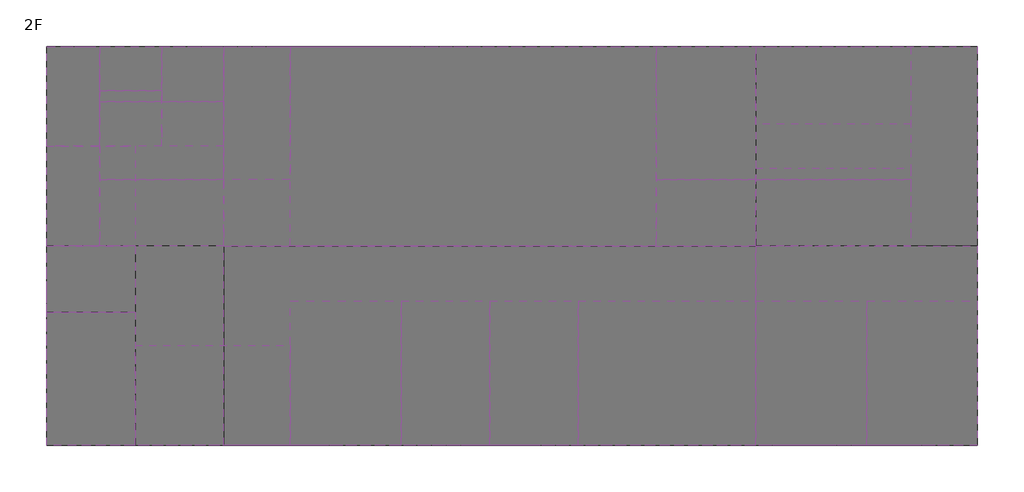
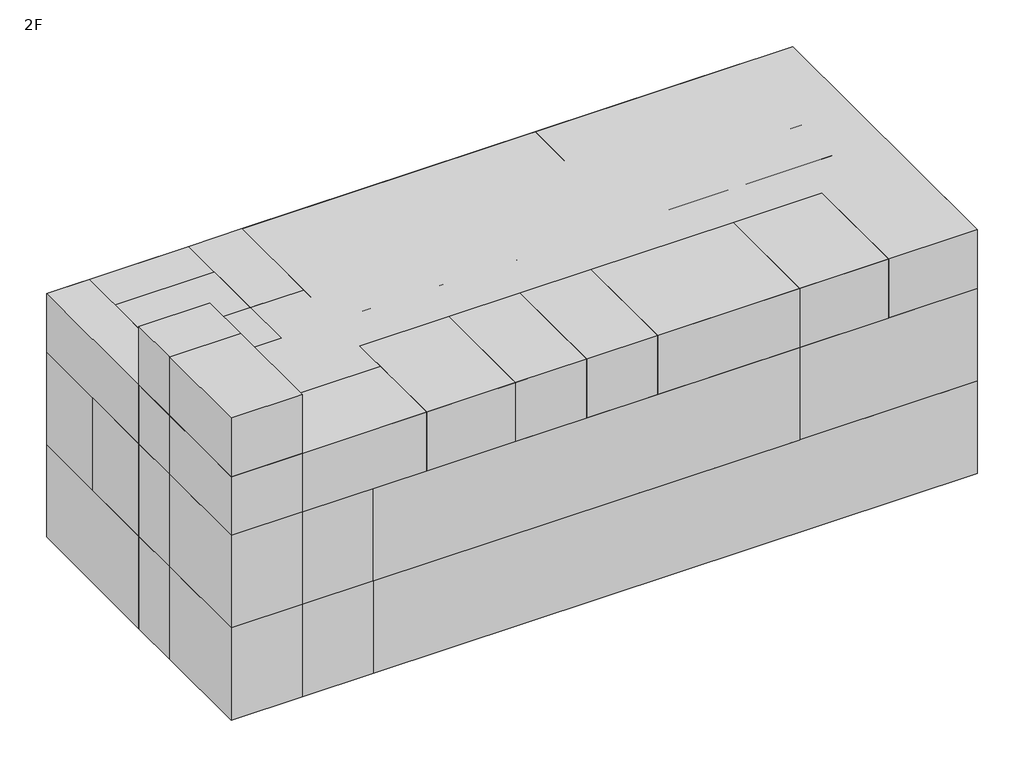
# One storey: 39 proxies.
"""IFC4 building model written with IfcOpenShell, lengths in millimetres."""

import ifcopenshell
import ifcopenshell.guid

model = None  # the IFC model being written
_history = None  # IfcOwnerHistory: only IFC2X3 demands one
_inside = {}  # id of a spatial element -> (the spatial element, [elements in it])
_under = {}  # id of a project, library or spatial element -> (it, [spatial elements below it])
_declared = {}  # id of a project -> (the project, [libraries it declares])
_typed = {}  # id of a type object -> (the type object, [elements of that type])
_made_of = {}  # id of a material, layer set ... -> (it, [elements and type objects made of it])


def new_model(schema):
    """Start an empty IFC model of exactly this schema.

    Asked for "IFC4X3", IfcOpenShell would pick the latest addendum, in which some entities
    have other attributes; the version numbers below select the first issue.
    IFC2X3 requires an IfcOwnerHistory on every rooted entity: one is made here for all.
    """
    global model, _history
    if schema == "IFC4X3":
        model = ifcopenshell.file(schema_version=(4, 3, 0, 0))
    else:
        model = ifcopenshell.file(schema=schema)
    _inside.clear()
    _under.clear()
    _declared.clear()
    _typed.clear()
    _made_of.clear()
    _history = None
    if model.schema == "IFC2X3":
        org = make("IfcOrganization", Name="unknown")
        user = make(
            "IfcPersonAndOrganization",
            ThePerson=make("IfcPerson", FamilyName="unknown"),
            TheOrganization=org,
        )
        app = make(
            "IfcApplication",
            ApplicationDeveloper=org,
            Version="unknown",
            ApplicationFullName="unknown",
            ApplicationIdentifier="unknown",
        )
        _history = make(
            "IfcOwnerHistory",
            OwningUser=user,
            OwningApplication=app,
            ChangeAction="ADDED",
            CreationDate=0,
        )
    return model


def make(cls, **values):
    """One entity of the class cls with the attributes given. An attribute that is None is left unset."""
    return model.create_entity(
        cls, **{name: value for name, value in values.items() if value is not None}
    )


def rooted(cls, **values):
    """An entity with a GlobalId (a new one), such as an element, a storey or a relation."""
    return make(cls, GlobalId=ifcopenshell.guid.new(), OwnerHistory=_history, **values)


def si_unit(unit_type, name, prefix=None):
    """IfcSIUnit, for example si_unit("LENGTHUNIT", "METRE", prefix="MILLI")."""
    return make("IfcSIUnit", UnitType=unit_type, Prefix=prefix, Name=name)


def assignment(units):
    """IfcUnitAssignment: the units of a project."""
    return None if units is None else make("IfcUnitAssignment", Units=units)


def point(xyz):
    """IfcCartesianPoint."""
    return None if xyz is None else make("IfcCartesianPoint", Coordinates=xyz)


def direction(xyz):
    """IfcDirection."""
    return None if xyz is None else make("IfcDirection", DirectionRatios=xyz)


def frame(location, z_axis=None, x_axis=None):
    """IfcAxis2Placement3D, a coordinate frame: its origin and axes. An axis left out is left unset."""
    return make(
        "IfcAxis2Placement3D",
        Location=point(location),
        Axis=direction(z_axis),
        RefDirection=direction(x_axis),
    )


def origin():
    """The frame at (0, 0, 0) with its axes left unset."""
    return frame((0.0, 0.0, 0.0))


def origin_with_axes():
    """The frame at (0, 0, 0) with the z axis (0, 0, 1) and the x axis (1, 0, 0) written out."""
    return frame((0.0, 0.0, 0.0), z_axis=(0.0, 0.0, 1.0), x_axis=(1.0, 0.0, 0.0))


def place(relative_to, where):
    """IfcLocalPlacement: puts the frame where relative to a parent placement (None: the world)."""
    return make(
        "IfcLocalPlacement", PlacementRelTo=relative_to, RelativePlacement=where
    )


def context(
    kind, dimensions, precision=None, world=None, true_north=None, identifier=None
):
    """IfcGeometricRepresentationContext, for example the 3D "Model" context."""
    return make(
        "IfcGeometricRepresentationContext",
        ContextIdentifier=identifier,
        ContextType=kind,
        CoordinateSpaceDimension=dimensions,
        Precision=precision,
        WorldCoordinateSystem=world,
        TrueNorth=true_north,
    )


def project(units=None, contexts=None):
    """IfcProject with its units and contexts."""
    return rooted(
        "IfcProject",
        Name="project",
        RepresentationContexts=contexts,
        UnitsInContext=assignment(units),
    )


def spatial(cls, under=None, at=None, **own):
    """A site, building, storey or space (cls), placed at a placement, below another one or the project."""
    s = rooted(cls, ObjectPlacement=at, **own)
    if under is not None:
        _under.setdefault(under.id(), (under, []))[1].append(s)
    return s


def polyline(points):
    """IfcPolyline through the points."""
    return make("IfcPolyline", Points=[point(p) for p in points])


def outline(outer, holes=None, kind="AREA"):
    """IfcArbitraryClosedProfileDef: a profile drawn as a closed curve; with holes, ...WithVoids."""
    if holes is None:
        return make("IfcArbitraryClosedProfileDef", ProfileType=kind, OuterCurve=outer)
    return make(
        "IfcArbitraryProfileDefWithVoids",
        ProfileType=kind,
        OuterCurve=outer,
        InnerCurves=holes,
    )


def extrude(swept, where, along, depth):
    """IfcExtrudedAreaSolid: the profile swept, set in the frame where, extruded along a direction by depth."""
    return make(
        "IfcExtrudedAreaSolid",
        SweptArea=swept,
        Position=where,
        ExtrudedDirection=direction(along),
        Depth=depth,
    )


def shape(context_of_items, identifier, shape_type, items):
    """IfcShapeRepresentation: the items that make up one representation, for example the "Body"."""
    return make(
        "IfcShapeRepresentation",
        ContextOfItems=context_of_items,
        RepresentationIdentifier=identifier,
        RepresentationType=shape_type,
        Items=items,
    )


def source(mapping_origin, context_of_items, identifier, shape_type, items):
    """IfcRepresentationMap: a shape defined once, which mapped items show again and again."""
    return make(
        "IfcRepresentationMap",
        MappingOrigin=mapping_origin,
        MappedRepresentation=shape(context_of_items, identifier, shape_type, items),
    )


def transform(
    local_origin,
    x_axis=None,
    y_axis=None,
    z_axis=None,
    scale=None,
    scale2=None,
    scale3=None,
    uniform=True,
):
    """IfcCartesianTransformationOperator3D, or its non-uniform kind. x_axis, y_axis, z_axis: its Axis1, 2, 3."""
    if uniform:
        return make(
            "IfcCartesianTransformationOperator3D",
            Axis1=direction(x_axis),
            Axis2=direction(y_axis),
            LocalOrigin=point(local_origin),
            Scale=scale,
            Axis3=direction(z_axis),
        )
    return make(
        "IfcCartesianTransformationOperator3DnonUniform",
        Axis1=direction(x_axis),
        Axis2=direction(y_axis),
        LocalOrigin=point(local_origin),
        Scale=scale,
        Axis3=direction(z_axis),
        Scale2=scale2,
        Scale3=scale3,
    )


def mapped(mapping_source, mapping_target):
    """IfcMappedItem: shows the shape of a source again, moved by a transform."""
    return make(
        "IfcMappedItem", MappingSource=mapping_source, MappingTarget=mapping_target
    )


def made_of(thing, what):
    """Note that an element or type object is made of a material, layer set ...; save() writes the relation."""
    if what is not None:
        _made_of.setdefault(what.id(), (what, []))[1].append(thing)
    return thing


def element(
    cls,
    number,
    at=None,
    inside=None,
    cuts=None,
    type_object=None,
    material=None,
    context=None,
    identifier="Body",
    shape_type=None,
    held_by="IfcProductDefinitionShape",
    body=None,
    shapes=None,
    **own,
):
    """One element of the class cls, such as IfcWall. Its Tag is "e" and its number.

    at: its placement. inside: the storey or other place that contains it. cuts: it is an
    opening in that element (IfcRelVoidsElement). A single representation is given by context,
    identifier, shape_type and body (its items); several are given by shapes. held_by: the class
    of the entity that holds the representations. save() writes the other relations.
    """
    e = rooted(cls, Tag="e%d" % number, ObjectPlacement=at, **own)
    if body is not None:
        shapes = [shape(context, identifier, shape_type, body)]
    if shapes is not None:
        e.Representation = make(held_by, Representations=shapes)
    if inside is not None:
        _inside.setdefault(inside.id(), (inside, []))[1].append(e)
    if cuts is not None:
        rooted(
            "IfcRelVoidsElement", RelatingBuildingElement=cuts, RelatedOpeningElement=e
        )
    if type_object is not None:
        _typed.setdefault(type_object.id(), (type_object, []))[1].append(e)
    return made_of(e, material)


def aggregate(whole, parts):
    """IfcRelAggregates: a whole, such as a stair, and the parts it consists of."""
    return rooted("IfcRelAggregates", RelatingObject=whole, RelatedObjects=parts)


def save(model, path):
    """Write the relations noted so far, then the file.

    IfcRelAggregates (storeys below a building ...), IfcRelContainedInSpatialStructure (elements
    in a storey), IfcRelDefinesByType, IfcRelAssociatesMaterial and IfcRelDeclares: one each for
    every whole, place, type object, material and project.
    """
    for whole, parts in _under.values():
        aggregate(whole, parts)
    for where, things in _inside.values():
        rooted(
            "IfcRelContainedInSpatialStructure",
            RelatedElements=things,
            RelatingStructure=where,
        )
    for kind, things in _typed.values():
        rooted("IfcRelDefinesByType", RelatedObjects=things, RelatingType=kind)
    for what, things in _made_of.values():
        rooted("IfcRelAssociatesMaterial", RelatedObjects=things, RelatingMaterial=what)
    for by, libraries in _declared.values():
        rooted("IfcRelDeclares", RelatingContext=by, RelatedDefinitions=libraries)
    model.write(path)


def generic_models_2d265e4a(model_context):
    return source(origin(), model_context, "Body", "SweptSolid", [
        extrude(outline(polyline([(4500.0, 5000.0), (4500.0, -5000.0), (-4500.0, -5000.0), (-4500.0, 5000.0), (4500.0, 5000.0)])), origin_with_axes(), (0.0, 0.0, 1.0), 5500.0),
    ])


def generic_models_8934d72c(model_context):
    return source(origin(), model_context, "Body", "SweptSolid", [
        extrude(outline(polyline([(2000.0, 4500.0), (2000.0, -4500.0), (-2000.0, -4500.0), (-2000.0, 4500.0), (2000.0, 4500.0)])), origin_with_axes(), (0.0, 0.0, 1.0), 5500.0),
    ])


def generic_models_626d8198(model_context):
    return source(origin(), model_context, "Body", "SweptSolid", [
        extrude(outline(polyline([(2000.0, 1500.0), (2000.0, -1500.0), (-2000.0, -1500.0), (-2000.0, 1500.0), (2000.0, 1500.0)])), origin_with_axes(), (0.0, 0.0, 1.0), 5500.0),
    ])


def generic_models_cc1dae17(model_context):
    return source(origin(), model_context, "Body", "SweptSolid", [
        extrude(outline(polyline([(2000.0, 3000.0), (2000.0, -3000.0), (-2000.0, -3000.0), (-2000.0, 3000.0), (2000.0, 3000.0)])), origin_with_axes(), (0.0, 0.0, 1.0), 5500.0),
    ])


def generic_models_7ea3b148(model_context):
    return source(origin(), model_context, "Body", "SweptSolid", [
        extrude(outline(polyline([(4500.0, 12000.0), (4500.0, -12000.0), (-4500.0, -12000.0), (-4500.0, 12000.0), (4500.0, 12000.0)])), origin_with_axes(), (0.0, 0.0, 1.0), 5500.0),
    ])


def generic_models_85ff21bb(model_context):
    return source(origin(), model_context, "Body", "SweptSolid", [
        extrude(outline(polyline([(3500.0, 1750.0), (3500.0, -1750.0), (-3500.0, -1750.0), (-3500.0, 1750.0), (3500.0, 1750.0)])), origin_with_axes(), (0.0, 0.0, 1.0), 5500.0),
    ])


def generic_models_570012e4(model_context):
    return source(origin(), model_context, "Body", "SweptSolid", [
        extrude(outline(polyline([(1200.0, 2250.0), (1200.0, -2250.0), (-1200.0, -2250.0), (-1200.0, 2250.0), (1200.0, 2250.0)])), origin_with_axes(), (0.0, 0.0, 1.0), 5500.0),
    ])


def generic_models_971c0b89(model_context):
    return source(origin(), model_context, "Body", "SweptSolid", [
        extrude(outline(polyline([(2000.0, 2250.0), (2000.0, -2250.0), (-2000.0, -2250.0), (-2000.0, 2250.0), (2000.0, 2250.0)])), origin_with_axes(), (0.0, 0.0, 1.0), 5500.0),
    ])


def generic_models_ac48a1a3(model_context):
    return source(origin(), model_context, "Body", "SweptSolid", [
        extrude(outline(polyline([(1400.0, 2250.0), (1400.0, -2250.0), (-1400.0, -2250.0), (-1400.0, 2250.0), (1400.0, 2250.0)])), origin_with_axes(), (0.0, 0.0, 1.0), 5500.0),
    ])


def generic_models_ee32b0c6(model_context):
    return source(origin(), model_context, "Body", "SweptSolid", [
        extrude(outline(polyline([(1400.0, 1000.0), (1400.0, -1000.0), (-1400.0, -1000.0), (-1400.0, 1000.0), (1400.0, 1000.0)])), origin_with_axes(), (0.0, 0.0, 1.0), 5500.0),
    ])


def generic_models_0ee3397c(model_context):
    return source(origin(), model_context, "Body", "SweptSolid", [
        extrude(outline(polyline([(1400.0, 1250.0), (1400.0, -1250.0), (-1400.0, -1250.0), (-1400.0, 1250.0), (1400.0, 1250.0)])), origin_with_axes(), (0.0, 0.0, 1.0), 5500.0),
    ])


def generic_models_8c4134a9(model_context):
    return source(origin(), model_context, "Body", "SweptSolid", [
        extrude(outline(polyline([(3250.0, 2000.0), (3250.0, -2000.0), (-3250.0, -2000.0), (-3250.0, 2000.0), (3250.0, 2000.0)])), origin_with_axes(), (0.0, 0.0, 1.0), 3500.0),
    ])


def generic_models_ccc8c8c2(model_context):
    return source(origin(), model_context, "Body", "SweptSolid", [
        extrude(outline(polyline([(3000.0, 5750.0), (3000.0, -5750.0), (-3000.0, -5750.0), (-3000.0, 5750.0), (3000.0, 5750.0)])), origin_with_axes(), (0.0, 0.0, 1.0), 3500.0),
    ])


def generic_models_70f6ae48(model_context):
    return source(origin(), model_context, "Body", "SweptSolid", [
        extrude(outline(polyline([(3250.0, 4000.0), (3250.0, -4000.0), (-3250.0, -4000.0), (-3250.0, 4000.0), (3250.0, 4000.0)])), origin_with_axes(), (0.0, 0.0, 1.0), 3500.0),
    ])


def generic_models_f0561c1d(model_context):
    return source(origin(), model_context, "Body", "SweptSolid", [
        extrude(outline(polyline([(4500.0, 8250.0), (4500.0, -8250.0), (-4500.0, -8250.0), (-4500.0, 8250.0), (4500.0, 8250.0)])), origin_with_axes(), (0.0, 0.0, 1.0), 3500.0),
    ])


def generic_models_249c6621(model_context):
    return source(origin(), model_context, "Body", "SweptSolid", [
        extrude(outline(polyline([(3250.0, 2500.0), (3250.0, -2500.0), (-3250.0, -2500.0), (-3250.0, 2500.0), (3250.0, 2500.0)])), origin_with_axes(), (0.0, 0.0, 1.0), 3500.0),
    ])


def generic_models_f1f4091a(model_context):
    return source(origin(), model_context, "Body", "SweptSolid", [
        extrude(outline(polyline([(1500.0, 5750.0), (1500.0, -5750.0), (-1500.0, -5750.0), (-1500.0, 5750.0), (1500.0, 5750.0)])), origin_with_axes(), (0.0, 0.0, 1.0), 3500.0),
    ])


def generic_models_10b6925f(model_context):
    return source(origin(), model_context, "Body", "SweptSolid", [
        extrude(outline(polyline([(2250.0, 3500.0), (2250.0, -3500.0), (-2250.0, -3500.0), (-2250.0, 3500.0), (2250.0, 3500.0)])), origin_with_axes(), (0.0, 0.0, 1.0), 3500.0),
    ])


def generic_models_b37916ea(model_context):
    return source(origin(), model_context, "Body", "SweptSolid", [
        extrude(outline(polyline([(1750.0, 2800.0), (1750.0, -2800.0), (-1750.0, -2800.0), (-1750.0, 2800.0), (1750.0, 2800.0)])), origin_with_axes(), (0.0, 0.0, 1.0), 3500.0),
    ])


def generic_models_6c75c912(model_context):
    return source(origin(), model_context, "Body", "SweptSolid", [
        extrude(outline(polyline([(1250.0, 2800.0), (1250.0, -2800.0), (-1250.0, -2800.0), (-1250.0, 2800.0), (1250.0, 2800.0)])), origin_with_axes(), (0.0, 0.0, 1.0), 3500.0),
    ])


def generic_models_a5818909(model_context):
    return source(origin(), model_context, "Body", "SweptSolid", [
        extrude(outline(polyline([(3000.0, 1500.0), (3000.0, -1500.0), (-3000.0, -1500.0), (-3000.0, 1500.0), (3000.0, 1500.0)])), origin_with_axes(), (0.0, 0.0, 1.0), 3500.0),
    ])


def generic_models_f42d0df8(model_context):
    return source(origin(), model_context, "Body", "SweptSolid", [
        extrude(outline(polyline([(1500.0, 2800.0), (1500.0, -2800.0), (-1500.0, -2800.0), (-1500.0, 2800.0), (1500.0, 2800.0)])), origin_with_axes(), (0.0, 0.0, 1.0), 3500.0),
    ])


def generic_models_4c644d41(model_context):
    return source(origin(), model_context, "Body", "SweptSolid", [
        extrude(outline(polyline([(2000.0, 1500.0), (2000.0, -1500.0), (-2000.0, -1500.0), (-2000.0, 1500.0), (2000.0, 1500.0)])), origin_with_axes(), (0.0, 0.0, 1.0), 3500.0),
    ])


def generic_models_c89eb543(model_context):
    return source(origin(), model_context, "Body", "SweptSolid", [
        extrude(outline(polyline([(2000.0, 3000.0), (2000.0, -3000.0), (-2000.0, -3000.0), (-2000.0, 3000.0), (2000.0, 3000.0)])), origin_with_axes(), (0.0, 0.0, 1.0), 3500.0),
    ])


def generic_models_3f6e5246(model_context):
    return source(origin(), model_context, "Body", "SweptSolid", [
        extrude(outline(polyline([(1200.0, 4500.0), (1200.0, -4500.0), (-1200.0, -4500.0), (-1200.0, 4500.0), (1200.0, 4500.0)])), origin_with_axes(), (0.0, 0.0, 1.0), 3500.0),
    ])


def generic_models_50f5a469(model_context):
    return source(origin(), model_context, "Body", "SweptSolid", [
        extrude(outline(polyline([(4500.0, 16000.0), (4500.0, -16000.0), (-4500.0, -16000.0), (-4500.0, 16000.0), (4500.0, 16000.0)])), origin_with_axes(), (0.0, 0.0, 1.0), 5500.0),
    ])


def generic_models_8b5775ea(model_context):
    return source(origin(), model_context, "Body", "SweptSolid", [
        extrude(outline(polyline([(4500.0, 17000.0), (4500.0, -17000.0), (-4500.0, -17000.0), (-4500.0, 17000.0), (4500.0, 17000.0)])), origin_with_axes(), (0.0, 0.0, 1.0), 5500.0),
    ])


def generic_models_3d03af35(model_context):
    return source(origin(), model_context, "Body", "SweptSolid", [
        extrude(outline(polyline([(21000.0, 9000.0), (21000.0, -9000.0), (-21000.0, -9000.0), (-21000.0, 9000.0), (21000.0, 9000.0)])), origin_with_axes(), (0.0, 0.0, 1.0), 5500.0),
    ])


def generic_models_bb515c93(model_context):
    return source(origin(), model_context, "Body", "SweptSolid", [
        extrude(outline(polyline([(9000.0, 21000.0), (9000.0, -21000.0), (-9000.0, -21000.0), (-9000.0, 21000.0), (9000.0, 21000.0)])), origin_with_axes(), (0.0, 0.0, 1.0), 3500.0),
    ])


model = new_model("IFC4")

# Units and contexts
model_context = context("Model", 3, world=origin())
ifc_project = project(units=[si_unit("LENGTHUNIT", "METRE", prefix="MILLI")], contexts=[model_context])

# Site, building, storey
site = spatial("IfcSite", under=ifc_project)
building = spatial("IfcBuilding", under=site)
storey = spatial("IfcBuildingStorey", under=building, Name="2F", Elevation=3500.0)

# Proxies
placement = place(None, origin())
generic_models_shape = generic_models_2d265e4a(model_context)
element("IfcBuildingElementProxy", 1, Name="Space Planning Box_hec : Space Planning Box_hec", ObjectType="Space Planning Box_hec : Space Planning Box_hec", at=placement, inside=storey, context=model_context, shape_type="MappedRepresentation", body=[
    mapped(generic_models_shape, transform((82459.6521483, 177423.8614395, 3500.0), x_axis=(0.0, 1.0, 0.0), y_axis=(-1.0, 0.0, 0.0), z_axis=(0.0, 0.0, 1.0))),
])
generic_models_2_shape = generic_models_8934d72c(model_context)
element("IfcBuildingElementProxy", 2, Name="Space Planning Box_hec : Space Planning Box_hec", ObjectType="Space Planning Box_hec : Space Planning Box_hec", at=placement, inside=storey, context=model_context, shape_type="MappedRepresentation", body=[
    mapped(generic_models_2_shape, transform((51459.6521483, 168423.8614395, 3500.0), x_axis=(1.0, 0.0, 0.0), y_axis=(0.0, 1.0, 0.0), z_axis=(0.0, 0.0, 1.0))),
])
generic_models_3_shape = generic_models_626d8198(model_context)
element("IfcBuildingElementProxy", 3, Name="Space Planning Box_hec : Space Planning Box_hec", ObjectType="Space Planning Box_hec : Space Planning Box_hec", at=placement, inside=storey, context=model_context, shape_type="MappedRepresentation", body=[
    mapped(generic_models_3_shape, transform((47459.6521483, 171423.8614395, 3500.0), x_axis=(1.0, 0.0, 0.0), y_axis=(0.0, 1.0, 0.0), z_axis=(0.0, 0.0, 1.0))),
])
element("IfcBuildingElementProxy", 4, Name="Space Planning Box_hec : Space Planning Box_hec", ObjectType="Space Planning Box_hec : Space Planning Box_hec", at=placement, inside=storey, context=model_context, shape_type="MappedRepresentation", body=[
    mapped(generic_models_3_shape, transform((47459.6521483, 171423.8614395, 9000.0), x_axis=(1.0, 0.0, 0.0), y_axis=(0.0, 1.0, 0.0), z_axis=(0.0, 0.0, 1.0))),
])
generic_models_4_shape = generic_models_cc1dae17(model_context)
element("IfcBuildingElementProxy", 5, Name="Space Planning Box_hec : Space Planning Box_hec", ObjectType="Space Planning Box_hec : Space Planning Box_hec", at=placement, inside=storey, context=model_context, shape_type="MappedRepresentation", body=[
    mapped(generic_models_4_shape, transform((47459.6521483, 166923.8614395, 3500.0), x_axis=(1.0, 0.0, 0.0), y_axis=(0.0, 1.0, 0.0), z_axis=(0.0, 0.0, 1.0))),
])
element("IfcBuildingElementProxy", 6, Name="Space Planning Box_hec : Space Planning Box_hec", ObjectType="Space Planning Box_hec : Space Planning Box_hec", at=placement, inside=storey, context=model_context, shape_type="MappedRepresentation", body=[
    mapped(generic_models_4_shape, transform((47459.6521483, 166923.8614395, 9000.0), x_axis=(1.0, 0.0, 0.0), y_axis=(0.0, 1.0, 0.0), z_axis=(0.0, 0.0, 1.0))),
])
generic_models_5_shape = generic_models_7ea3b148(model_context)
element("IfcBuildingElementProxy", 7, Name="Space Planning Box_hec : Space Planning Box_hec", ObjectType="Space Planning Box_hec : Space Planning Box_hec", at=placement, inside=storey, context=model_context, shape_type="MappedRepresentation", body=[
    mapped(generic_models_5_shape, transform((65459.6521483, 177423.8614395, 9000.0), x_axis=(0.0, -1.0, 0.0), y_axis=(1.0, 0.0, 0.0), z_axis=(0.0, 0.0, 1.0))),
])
element("IfcBuildingElementProxy", 8, Name="Space Planning Box_hec : Space Planning Box_hec", ObjectType="Space Planning Box_hec : Space Planning Box_hec", at=placement, inside=storey, context=model_context, shape_type="MappedRepresentation", body=[
    mapped(generic_models_5_shape, transform((65459.6521483, 168423.8614395, 9000.0), x_axis=(0.0, -1.0, 0.0), y_axis=(1.0, 0.0, 0.0), z_axis=(0.0, 0.0, 1.0))),
])
generic_models_6_shape = generic_models_85ff21bb(model_context)
element("IfcBuildingElementProxy", 9, Name="Space Planning Box_hec : Space Planning Box_hec", ObjectType="Space Planning Box_hec : Space Planning Box_hec", at=placement, inside=storey, context=model_context, shape_type="MappedRepresentation", body=[
    mapped(generic_models_6_shape, transform((80959.6521483, 180173.8614395, 9000.0), x_axis=(1.0, 0.0, 0.0), y_axis=(0.0, 1.0, 0.0), z_axis=(0.0, 0.0, 1.0))),
])
element("IfcBuildingElementProxy", 10, Name="Space Planning Box_hec : Space Planning Box_hec", ObjectType="Space Planning Box_hec : Space Planning Box_hec", at=placement, inside=storey, context=model_context, shape_type="MappedRepresentation", body=[
    mapped(generic_models_shape, transform((82459.6521483, 168423.8614395, 9000.0), x_axis=(0.0, 1.0, 0.0), y_axis=(-1.0, 0.0, 0.0), z_axis=(0.0, 0.0, 1.0))),
])
element("IfcBuildingElementProxy", 11, Name="Space Planning Box_hec : Space Planning Box_hec", ObjectType="Space Planning Box_hec : Space Planning Box_hec", at=placement, inside=storey, context=model_context, shape_type="MappedRepresentation", body=[
    mapped(generic_models_6_shape, transform((80959.6521483, 174673.8614395, 9000.0), x_axis=(1.0, 0.0, 0.0), y_axis=(0.0, 1.0, 0.0), z_axis=(0.0, 0.0, 1.0))),
])
generic_models_7_shape = generic_models_570012e4(model_context)
element("IfcBuildingElementProxy", 12, Name="Space Planning Box_hec : Space Planning Box_hec", ObjectType="Space Planning Box_hec : Space Planning Box_hec", at=placement, inside=storey, context=model_context, shape_type="MappedRepresentation", body=[
    mapped(generic_models_7_shape, transform((46659.6521483, 179673.8614395, 9000.0), x_axis=(1.0, 0.0, 0.0), y_axis=(0.0, 1.0, 0.0), z_axis=(0.0, 0.0, 1.0))),
])
generic_models_8_shape = generic_models_971c0b89(model_context)
element("IfcBuildingElementProxy", 13, Name="Space Planning Box_hec : Space Planning Box_hec", ObjectType="Space Planning Box_hec : Space Planning Box_hec", at=placement, inside=storey, context=model_context, shape_type="MappedRepresentation", body=[
    mapped(generic_models_8_shape, transform((47459.6521483, 175173.8614395, 9000.0), x_axis=(1.0, 0.0, 0.0), y_axis=(0.0, 1.0, 0.0), z_axis=(0.0, 0.0, 1.0))),
])
generic_models_9_shape = generic_models_ac48a1a3(model_context)
element("IfcBuildingElementProxy", 14, Name="Space Planning Box_hec : Space Planning Box_hec", ObjectType="Space Planning Box_hec : Space Planning Box_hec", at=placement, inside=storey, context=model_context, shape_type="MappedRepresentation", body=[
    mapped(generic_models_9_shape, transform((52059.6521483, 179673.8614395, 9000.0), x_axis=(1.0, 0.0, 0.0), y_axis=(0.0, 1.0, 0.0), z_axis=(0.0, 0.0, 1.0))),
])
generic_models_10_shape = generic_models_ee32b0c6(model_context)
element("IfcBuildingElementProxy", 15, Name="Space Planning Box_hec : Space Planning Box_hec", ObjectType="Space Planning Box_hec : Space Planning Box_hec", at=placement, inside=storey, context=model_context, shape_type="MappedRepresentation", body=[
    mapped(generic_models_10_shape, transform((49259.6521483, 180923.8614395, 9000.0), x_axis=(1.0, 0.0, 0.0), y_axis=(0.0, 1.0, 0.0), z_axis=(0.0, 0.0, 1.0))),
])
generic_models_11_shape = generic_models_0ee3397c(model_context)
element("IfcBuildingElementProxy", 16, Name="Space Planning Box_hec : Space Planning Box_hec", ObjectType="Space Planning Box_hec : Space Planning Box_hec", at=placement, inside=storey, context=model_context, shape_type="MappedRepresentation", body=[
    mapped(generic_models_11_shape, transform((49259.6521483, 178673.8614395, 9000.0), x_axis=(1.0, 0.0, 0.0), y_axis=(0.0, 1.0, 0.0), z_axis=(0.0, 0.0, 1.0))),
])
generic_models_12_shape = generic_models_8c4134a9(model_context)
element("IfcBuildingElementProxy", 17, Name="Space Planning Box_hec : Space Planning Box_hec", ObjectType="Space Planning Box_hec : Space Planning Box_hec", at=placement, inside=storey, context=model_context, shape_type="MappedRepresentation", body=[
    mapped(generic_models_12_shape, transform((63459.6521483, 167173.8614395, 14500.0), x_axis=(0.0, 1.0, 0.0), y_axis=(-1.0, 0.0, 0.0), z_axis=(0.0, 0.0, 1.0))),
])
element("IfcBuildingElementProxy", 18, Name="Space Planning Box_hec : Space Planning Box_hec", ObjectType="Space Planning Box_hec : Space Planning Box_hec", at=placement, inside=storey, context=model_context, shape_type="MappedRepresentation", body=[
    mapped(generic_models_12_shape, transform((67459.6521483, 167173.8614395, 14500.0), x_axis=(0.0, 1.0, 0.0), y_axis=(-1.0, 0.0, 0.0), z_axis=(0.0, 0.0, 1.0))),
])
generic_models_13_shape = generic_models_ccc8c8c2(model_context)
element("IfcBuildingElementProxy", 19, Name="Space Planning Box_hec : Space Planning Box_hec", ObjectType="Space Planning Box_hec : Space Planning Box_hec", at=placement, inside=storey, context=model_context, shape_type="MappedRepresentation", body=[
    mapped(generic_models_13_shape, transform((78709.6521483, 178923.8614395, 14500.0), x_axis=(0.0, -1.0, 0.0), y_axis=(1.0, 0.0, 0.0), z_axis=(0.0, 0.0, 1.0))),
])
generic_models_14_shape = generic_models_70f6ae48(model_context)
element("IfcBuildingElementProxy", 20, Name="Space Planning Box_hec : Space Planning Box_hec", ObjectType="Space Planning Box_hec : Space Planning Box_hec", at=placement, inside=storey, context=model_context, shape_type="MappedRepresentation", body=[
    mapped(generic_models_14_shape, transform((73459.6521483, 167173.8614395, 14500.0), x_axis=(0.0, -1.0, 0.0), y_axis=(1.0, 0.0, 0.0), z_axis=(0.0, 0.0, 1.0))),
])
generic_models_15_shape = generic_models_f0561c1d(model_context)
element("IfcBuildingElementProxy", 21, Name="Space Planning Box_hec : Space Planning Box_hec", ObjectType="Space Planning Box_hec : Space Planning Box_hec", at=placement, inside=storey, context=model_context, shape_type="MappedRepresentation", body=[
    mapped(generic_models_15_shape, transform((64709.6521483, 177423.8614395, 14500.0), x_axis=(0.0, -1.0, 0.0), y_axis=(1.0, 0.0, 0.0), z_axis=(0.0, 0.0, 1.0))),
])
generic_models_16_shape = generic_models_249c6621(model_context)
element("IfcBuildingElementProxy", 22, Name="Space Planning Box_hec : Space Planning Box_hec", ObjectType="Space Planning Box_hec : Space Planning Box_hec", at=placement, inside=storey, context=model_context, shape_type="MappedRepresentation", body=[
    mapped(generic_models_16_shape, transform((79959.6521483, 167173.8614395, 14500.0), x_axis=(0.0, -1.0, 0.0), y_axis=(1.0, 0.0, 0.0), z_axis=(0.0, 0.0, 1.0))),
])
element("IfcBuildingElementProxy", 23, Name="Space Planning Box_hec : Space Planning Box_hec", ObjectType="Space Planning Box_hec : Space Planning Box_hec", at=placement, inside=storey, context=model_context, shape_type="MappedRepresentation", body=[
    mapped(generic_models_16_shape, transform((58959.6521483, 167173.8614395, 14500.0), x_axis=(0.0, 1.0, 0.0), y_axis=(-1.0, 0.0, 0.0), z_axis=(0.0, 0.0, 1.0))),
])
element("IfcBuildingElementProxy", 24, Name="Space Planning Box_hec : Space Planning Box_hec", ObjectType="Space Planning Box_hec : Space Planning Box_hec", at=placement, inside=storey, context=model_context, shape_type="MappedRepresentation", body=[
    mapped(generic_models_16_shape, transform((84959.6521483, 167173.8614395, 14500.0), x_axis=(0.0, 1.0, 0.0), y_axis=(-1.0, 0.0, 0.0), z_axis=(0.0, 0.0, 1.0))),
])
generic_models_17_shape = generic_models_f1f4091a(model_context)
element("IfcBuildingElementProxy", 25, Name="Space Planning Box_hec : Space Planning Box_hec", ObjectType="Space Planning Box_hec : Space Planning Box_hec", at=placement, inside=storey, context=model_context, shape_type="MappedRepresentation", body=[
    mapped(generic_models_17_shape, transform((78709.6521483, 174423.8614395, 14500.0), x_axis=(0.0, 1.0, 0.0), y_axis=(-1.0, 0.0, 0.0), z_axis=(0.0, 0.0, 1.0))),
])
generic_models_18_shape = generic_models_10b6925f(model_context)
element("IfcBuildingElementProxy", 26, Name="Space Planning Box_hec : Space Planning Box_hec", ObjectType="Space Planning Box_hec : Space Planning Box_hec", at=placement, inside=storey, context=model_context, shape_type="MappedRepresentation", body=[
    mapped(generic_models_18_shape, transform((52959.6521483, 166173.8614395, 14500.0), x_axis=(0.0, -1.0, 0.0), y_axis=(1.0, 0.0, 0.0), z_axis=(0.0, 0.0, 1.0))),
])
generic_models_19_shape = generic_models_b37916ea(model_context)
element("IfcBuildingElementProxy", 27, Name="Space Planning Box_hec : Space Planning Box_hec", ObjectType="Space Planning Box_hec : Space Planning Box_hec", at=placement, inside=storey, context=model_context, shape_type="MappedRepresentation", body=[
    mapped(generic_models_19_shape, transform((50659.6521483, 177673.8614395, 14500.0), x_axis=(0.0, -1.0, 0.0), y_axis=(1.0, 0.0, 0.0), z_axis=(0.0, 0.0, 1.0))),
])
generic_models_20_shape = generic_models_6c75c912(model_context)
element("IfcBuildingElementProxy", 28, Name="Space Planning Box_hec : Space Planning Box_hec", ObjectType="Space Planning Box_hec : Space Planning Box_hec", at=placement, inside=storey, context=model_context, shape_type="MappedRepresentation", body=[
    mapped(generic_models_20_shape, transform((50659.6521483, 180673.8614395, 14500.0), x_axis=(0.0, -1.0, 0.0), y_axis=(1.0, 0.0, 0.0), z_axis=(0.0, 0.0, 1.0))),
])
generic_models_21_shape = generic_models_a5818909(model_context)
element("IfcBuildingElementProxy", 29, Name="Space Planning Box_hec : Space Planning Box_hec", ObjectType="Space Planning Box_hec : Space Planning Box_hec", at=placement, inside=storey, context=model_context, shape_type="MappedRepresentation", body=[
    mapped(generic_models_21_shape, transform((54959.6521483, 178923.8614395, 14500.0), x_axis=(0.0, -1.0, 0.0), y_axis=(1.0, 0.0, 0.0), z_axis=(0.0, 0.0, 1.0))),
])
generic_models_22_shape = generic_models_f42d0df8(model_context)
element("IfcBuildingElementProxy", 30, Name="Space Planning Box_hec : Space Planning Box_hec", ObjectType="Space Planning Box_hec : Space Planning Box_hec", at=placement, inside=storey, context=model_context, shape_type="MappedRepresentation", body=[
    mapped(generic_models_22_shape, transform((50659.6521483, 174423.8614395, 14500.0), x_axis=(0.0, -1.0, 0.0), y_axis=(1.0, 0.0, 0.0), z_axis=(0.0, 0.0, 1.0))),
])
generic_models_23_shape = generic_models_4c644d41(model_context)
element("IfcBuildingElementProxy", 31, Name="Space Planning Box_hec : Space Planning Box_hec", ObjectType="Space Planning Box_hec : Space Planning Box_hec", at=placement, inside=storey, context=model_context, shape_type="MappedRepresentation", body=[
    mapped(generic_models_23_shape, transform((47459.6521483, 171423.8614395, 14500.0), x_axis=(1.0, 0.0, 0.0), y_axis=(0.0, 1.0, 0.0), z_axis=(0.0, 0.0, 1.0))),
])
element("IfcBuildingElementProxy", 32, Name="Space Planning Box_hec : Space Planning Box_hec", ObjectType="Space Planning Box_hec : Space Planning Box_hec", at=placement, inside=storey, context=model_context, shape_type="MappedRepresentation", body=[
    mapped(generic_models_23_shape, transform((47459.6521483, 171423.8614395, 18000.0), x_axis=(1.0, 0.0, 0.0), y_axis=(0.0, 1.0, 0.0), z_axis=(0.0, 0.0, 1.0))),
])
generic_models_24_shape = generic_models_c89eb543(model_context)
element("IfcBuildingElementProxy", 33, Name="Space Planning Box_hec : Space Planning Box_hec", ObjectType="Space Planning Box_hec : Space Planning Box_hec", at=placement, inside=storey, context=model_context, shape_type="MappedRepresentation", body=[
    mapped(generic_models_24_shape, transform((47459.6521483, 166923.8614395, 14500.0), x_axis=(1.0, 0.0, 0.0), y_axis=(0.0, 1.0, 0.0), z_axis=(0.0, 0.0, 1.0))),
])
element("IfcBuildingElementProxy", 34, Name="Space Planning Box_hec : Space Planning Box_hec", ObjectType="Space Planning Box_hec : Space Planning Box_hec", at=placement, inside=storey, context=model_context, shape_type="MappedRepresentation", body=[
    mapped(generic_models_24_shape, transform((47459.6521483, 166923.8614395, 18000.0), x_axis=(1.0, 0.0, 0.0), y_axis=(0.0, 1.0, 0.0), z_axis=(0.0, 0.0, 1.0))),
])
generic_models_25_shape = generic_models_3f6e5246(model_context)
element("IfcBuildingElementProxy", 35, Name="Space Planning Box_hec : Space Planning Box_hec", ObjectType="Space Planning Box_hec : Space Planning Box_hec", at=placement, inside=storey, context=model_context, shape_type="MappedRepresentation", body=[
    mapped(generic_models_25_shape, transform((46659.6521483, 177423.8614395, 14500.0), x_axis=(1.0, 0.0, 0.0), y_axis=(0.0, 1.0, 0.0), z_axis=(0.0, 0.0, 1.0))),
])
generic_models_26_shape = generic_models_50f5a469(model_context)
element("IfcBuildingElementProxy", 36, Name="Space Planning Box_hec : Space Planning Box_hec", ObjectType="Space Planning Box_hec : Space Planning Box_hec", at=placement, inside=storey, context=model_context, shape_type="MappedRepresentation", body=[
    mapped(generic_models_26_shape, transform((61459.6521483, 177423.8614395, 3500.0), x_axis=(0.0, 1.0, 0.0), y_axis=(-1.0, 0.0, 0.0), z_axis=(0.0, 0.0, 1.0))),
])
generic_models_27_shape = generic_models_8b5775ea(model_context)
element("IfcBuildingElementProxy", 37, Name="Space Planning Box_hec : Space Planning Box_hec", ObjectType="Space Planning Box_hec : Space Planning Box_hec", at=placement, inside=storey, context=model_context, shape_type="MappedRepresentation", body=[
    mapped(generic_models_27_shape, transform((70459.6521483, 168423.8614395, 3500.0), x_axis=(0.0, 1.0, 0.0), y_axis=(-1.0, 0.0, 0.0), z_axis=(0.0, 0.0, 1.0))),
])
generic_models_28_shape = generic_models_3d03af35(model_context)
element("IfcBuildingElementProxy", 38, Name="Space Planning Box_hec : Space Planning Box_hec", ObjectType="Space Planning Box_hec : Space Planning Box_hec", at=placement, inside=storey, context=model_context, shape_type="MappedRepresentation", body=[
    mapped(generic_models_28_shape, transform((66459.6521483, 172923.8614395, 9000.0), x_axis=(1.0, 0.0, 0.0), y_axis=(0.0, 1.0, 0.0), z_axis=(0.0, 0.0, 1.0))),
])
generic_models_29_shape = generic_models_bb515c93(model_context)
element("IfcBuildingElementProxy", 39, Name="Space Planning Box_hec : Space Planning Box_hec", ObjectType="Space Planning Box_hec : Space Planning Box_hec", at=placement, inside=storey, context=model_context, shape_type="MappedRepresentation", body=[
    mapped(generic_models_29_shape, transform((66459.6521483, 172923.8614395, 14500.0), x_axis=(0.0, -1.0, 0.0), y_axis=(1.0, 0.0, 0.0), z_axis=(0.0, 0.0, 1.0))),
])

save(model, "model.ifc")

# Revit data of these elements
# Type "Space Planning Box_hec : Space Planning Box_hec"
#   Type Comments = "..."
#   Room Name [instance default] = "?"
#   Interior Finish [instance default] = ""
#   Exterior Finish [instance default] = ""
#   Department [instance default] = ""
#   Assembly Code = "..."
#   Width [instance default] = 1524 mm
#   Program Area [instance default] = 0.00 m²
#   Length [instance default] = 1524 mm
#   Height [instance default] = 1524 mm
#   Area [instance default] = 2.32258 m²
#   Fill Color [instance default] = Cyan
#   Default Elevation = 0
# Element 1 (IfcBuildingElementProxy, "Space Planning Box_hec : Space Planning Box_hec")
#   Room Name = "Electrical Room (GIS)"
#   Interior Finish = "IW5..N/A..N/A,,WK1..N/A,,FL1,,CL1..N/A"
#   Exterior Finish = "N/A..N/A,,EW1..EW2..N/A"
#   Department = "AR"
#   Width = 9000 mm
#   Program Area = 90.00 m²
#   Length = 10000 mm
#   Height = 5500 mm
#   Area = 90.00 m²
#   Fill Color = Cyan
#   Phase Created = New Construction
#   Materials on its faces: "Cyan"
# Element 2 (IfcBuildingElementProxy, "Space Planning Box_hec : Space Planning Box_hec")
#   Room Name = "Lobby"
#   Interior Finish = "IW5..N/A..N/A,,WK3..N/A,,FL2,,CL3..N/A"
#   Exterior Finish = "N/A..N/A,,EW2..N/A..N/A"
#   Department = "AR"
#   Width = 4000 mm
#   Program Area = 36.00 m²
#   Length = 9000 mm
#   Height = 5500 mm
#   Area = 36.00 m²
#   Fill Color = Cyan
#   Phase Created = New Construction
#   Materials on its faces: "Cyan"
# Elements 3, 4 (IfcBuildingElementProxy, "Space Planning Box_hec : Space Planning Box_hec")
#   Room Name = "Elevator"
#   Interior Finish = "N/A..N/A..N/A,,N/A..N/A,,,,N/A..N/A"
#   Exterior Finish = "N/A..N/A,,EW2..N/A..N/A"
#   Department = "PATHV2"
#   Width = 4000 mm
#   Program Area = 12.00 m²
#   Length = 3000 mm
#   Height = 5500 mm
#   Area = 12.00 m²
#   Fill Color = Blue
#   Phase Created = New Construction
#   Materials on its faces: "Blue"
# Elements 5, 6 (IfcBuildingElementProxy, "Space Planning Box_hec : Space Planning Box_hec")
#   Room Name = "Staircase"
#   Interior Finish = "IW5..N/A..N/A,,WK3..N/A,,FL2,,CL1..N/A"
#   Exterior Finish = "N/A..N/A,,EW2..N/A..N/A"
#   Department = "PATHV1"
#   Width = 4000 mm
#   Program Area = 24.00 m²
#   Length = 6000 mm
#   Height = 5500 mm
#   Area = 24.00 m²
#   Fill Color = Green
#   Phase Created = New Construction
#   Materials on its faces: "Green"
# Element 7 (IfcBuildingElementProxy, "Space Planning Box_hec : Space Planning Box_hec")
#   Room Name = "Central Control Room"
#   Interior Finish = "IW5..N/A..N/A,,N/A..N/A,,FL5,,CL3..N/A"
#   Exterior Finish = "N/A..N/A,,EW1..N/A..N/A"
#   Department = "CI"
#   Width = 9000 mm
#   Program Area = 216.00 m²
#   Length = 24000 mm
#   Height = 5500 mm
#   Area = 216.00 m²
#   Fill Color = Yellow
#   Phase Created = New Construction
#   Materials on its faces: "Yellow"
# Element 8 (IfcBuildingElementProxy, "Space Planning Box_hec : Space Planning Box_hec")
#   Room Name = "Electronic Room"
#   Interior Finish = "IW5..N/A..N/A,,N/A..N/A,,FL5,,CL3..N/A"
#   Exterior Finish = "N/A..N/A,,EW1..N/A..N/A"
#   Department = "CI"
#   Width = 9000 mm
#   Program Area = 216.00 m²
#   Length = 24000 mm
#   Height = 5500 mm
#   Area = 216.00 m²
#   Fill Color = Yellow
#   Phase Created = New Construction
#   Materials on its faces: "Yellow"
# Element 9 (IfcBuildingElementProxy, "Space Planning Box_hec : Space Planning Box_hec")
#   Room Name = "Computer Room"
#   Interior Finish = "IW5..N/A..N/A,,N/A..N/A,,FL5,,CL3..N/A"
#   Exterior Finish = "N/A..N/A,,EW2..N/A..N/A"
#   Department = "AR"
#   Width = 7000 mm
#   Program Area = 24.50 m²
#   Length = 3500 mm
#   Height = 5500 mm
#   Area = 24.50 m²
#   Fill Color = Cyan
#   Phase Created = New Construction
#   Materials on its faces: "Cyan"
# Element 10 (IfcBuildingElementProxy, "Space Planning Box_hec : Space Planning Box_hec")
#   Room Name = "Electrical Room -3"
#   Interior Finish = "IW5..N/A..N/A,,N/A..N/A,,FL5,,CL3..N/A"
#   Exterior Finish = "N/A..N/A,,EW2..N/A..N/A"
#   Department = "EL"
#   Width = 9000 mm
#   Program Area = 90.00 m²
#   Length = 10000 mm
#   Height = 5500 mm
#   Area = 90.00 m²
#   Fill Color = Orange
#   Phase Created = New Construction
#   Materials on its faces: "Orange"
# Element 11 (IfcBuildingElementProxy, "Space Planning Box_hec : Space Planning Box_hec")
#   Room Name = "Communication Room"
#   Interior Finish = "IW5..N/A..N/A,,N/A..N/A,,FL5,,CL3..N/A"
#   Exterior Finish = "N/A..N/A,,N/A..N/A..N/A"
#   Department = "CI"
#   Width = 7000 mm
#   Program Area = 24.50 m²
#   Length = 3500 mm
#   Height = 5500 mm
#   Area = 24.50 m²
#   Fill Color = Yellow
#   Phase Created = New Construction
#   Materials on its faces: "Yellow"
# Element 12 (IfcBuildingElementProxy, "Space Planning Box_hec : Space Planning Box_hec")
#   Room Name = "Duct Shaft"
#   Interior Finish = "N/A..N/A..N/A,,N/A..N/A,,,,N/A..N/A"
#   Exterior Finish = "N/A..N/A,,EW2..N/A..N/A"
#   Department = "PATHV3"
#   Width = 2400 mm
#   Program Area = 10.80 m²
#   Length = 4500 mm
#   Height = 5500 mm
#   Area = 10.80 m²
#   Fill Color = Lavender
#   Phase Created = New Construction
#   Materials on its faces: "Lavender"
# Element 13 (IfcBuildingElementProxy, "Space Planning Box_hec : Space Planning Box_hec")
#   Room Name = "Toilet (M)"
#   Interior Finish = "IW3..N/A..N/A,,N/A..N/A,,FL3,,CL4..N/A"
#   Exterior Finish = "N/A..N/A,,EW2..N/A..N/A"
#   Department = "AR"
#   Width = 4000 mm
#   Program Area = 18.00 m²
#   Length = 4500 mm
#   Height = 5500 mm
#   Area = 18.00 m²
#   Fill Color = Cyan
#   Phase Created = New Construction
#   Materials on its faces: "Cyan"
# Element 14 (IfcBuildingElementProxy, "Space Planning Box_hec : Space Planning Box_hec")
#   Room Name = "Toilet"
#   Interior Finish = "IW3..N/A..N/A,,N/A..N/A,,FL3,,CL4..N/A"
#   Exterior Finish = "N/A..N/A,,EW2..N/A..N/A"
#   Department = "AR"
#   Width = 2800 mm
#   Program Area = 12.60 m²
#   Length = 4500 mm
#   Height = 5500 mm
#   Area = 12.60 m²
#   Fill Color = Cyan
#   Phase Created = New Construction
#   Materials on its faces: "Cyan"
# Element 15 (IfcBuildingElementProxy, "Space Planning Box_hec : Space Planning Box_hec")
#   Room Name = "Shower"
#   Interior Finish = "IW3..N/A..N/A,,N/A..N/A,,FL3,,CL4..N/A"
#   Exterior Finish = "N/A..N/A,,EW2..N/A..N/A"
#   Department = "AR"
#   Width = 2800 mm
#   Program Area = 5.60 m²
#   Length = 2000 mm
#   Height = 5500 mm
#   Area = 5.60 m²
#   Fill Color = Cyan
#   Phase Created = New Construction
#   Materials on its faces: "Cyan"
# Element 16 (IfcBuildingElementProxy, "Space Planning Box_hec : Space Planning Box_hec")
#   Room Name = "Locker(F)"
#   Interior Finish = "IW5..N/A..N/A,,WK3..N/A,,FL2,,CL3..N/A"
#   Exterior Finish = "N/A..N/A,,N/A..N/A..N/A"
#   Department = "AR"
#   Width = 2800 mm
#   Program Area = 7.00 m²
#   Length = 2500 mm
#   Height = 5500 mm
#   Area = 7.00 m²
#   Fill Color = Cyan
#   Phase Created = New Construction
#   Materials on its faces: "Cyan"
# Element 17 (IfcBuildingElementProxy, "Space Planning Box_hec : Space Planning Box_hec")
#   Room Name = "Manager Office-1"
#   Interior Finish = "IW5..N/A..N/A,,WK3..N/A,,FL2,,CL3..N/A"
#   Exterior Finish = "RF1..N/A,,EW1..N/A..N/A"
#   Department = "AR"
#   Width = 6500 mm
#   Program Area = 26.00 m²
#   Length = 4000 mm
#   Height = 3500 mm
#   Area = 26.00 m²
#   Fill Color = Cyan
#   Phase Created = New Construction
#   Materials on its faces: "Cyan"
# Element 18 (IfcBuildingElementProxy, "Space Planning Box_hec : Space Planning Box_hec")
#   Room Name = "Manager Office-2"
#   Interior Finish = "IW5..N/A..N/A,,WK3..N/A,,FL2,,CL3..N/A"
#   Exterior Finish = "RF1..N/A,,EW1..N/A..N/A"
#   Department = "AR"
#   Width = 6500 mm
#   Program Area = 26.00 m²
#   Length = 4000 mm
#   Height = 3500 mm
#   Area = 26.00 m²
#   Fill Color = Cyan
#   Phase Created = New Construction
#   Materials on its faces: "Cyan"
# Element 19 (IfcBuildingElementProxy, "Space Planning Box_hec : Space Planning Box_hec")
#   Room Name = "Meeting Room-1"
#   Interior Finish = "IW5..N/A..N/A,,WK3..N/A,,FL2,,CL3..N/A"
#   Exterior Finish = "RF1..N/A,,EW1..EW2..N/A"
#   Department = "AR"
#   Width = 6000 mm
#   Program Area = 69.00 m²
#   Length = 11500 mm
#   Height = 3500 mm
#   Area = 69.00 m²
#   Fill Color = Cyan
#   Phase Created = New Construction
#   Materials on its faces: "Cyan"
# Element 20 (IfcBuildingElementProxy, "Space Planning Box_hec : Space Planning Box_hec")
#   Room Name = "Meeting Room-2"
#   Interior Finish = "IW5..N/A..N/A,,WK3..N/A,,FL2,,CL3..N/A"
#   Exterior Finish = "RF1..N/A,,EW1..N/A..N/A"
#   Department = "AR"
#   Width = 6500 mm
#   Program Area = 52.00 m²
#   Length = 8000 mm
#   Height = 3500 mm
#   Area = 52.00 m²
#   Fill Color = Cyan
#   Phase Created = New Construction
#   Materials on its faces: "Cyan"
# Element 21 (IfcBuildingElementProxy, "Space Planning Box_hec : Space Planning Box_hec")
#   Room Name = "Open Office"
#   Interior Finish = "IW5..N/A..N/A,,WK3..N/A,,FL2,,CL3..N/A"
#   Exterior Finish = "RF1..N/A,,EW1..N/A..N/A"
#   Department = "HV"
#   Width = 9000 mm
#   Program Area = 148.50 m²
#   Length = 16500 mm
#   Height = 3500 mm
#   Area = 148.50 m²
#   Fill Color = Lime
#   Phase Created = New Construction
#   Materials on its faces: "Lime"
# Element 22 (IfcBuildingElementProxy, "Space Planning Box_hec : Space Planning Box_hec")
#   Room Name = "Office-1"
#   Interior Finish = "IW5..N/A..N/A,,WK3..N/A,,FL2,,CL3..N/A"
#   Exterior Finish = "RF1..N/A,,EW2..N/A..N/A"
#   Department = "AR"
#   Width = 6500 mm
#   Program Area = 32.50 m²
#   Length = 5000 mm
#   Height = 3500 mm
#   Area = 32.50 m²
#   Fill Color = Cyan
#   Phase Created = New Construction
#   Materials on its faces: "Cyan"
# Element 23 (IfcBuildingElementProxy, "Space Planning Box_hec : Space Planning Box_hec")
#   Room Name = "Storage"
#   Interior Finish = "IW5..N/A..N/A,,WK3..N/A,,FL2,,CL3..N/A"
#   Exterior Finish = "RF1..N/A,,EW1..N/A..N/A"
#   Department = "AR"
#   Width = 6500 mm
#   Program Area = 32.50 m²
#   Length = 5000 mm
#   Height = 3500 mm
#   Area = 32.50 m²
#   Fill Color = Cyan
#   Phase Created = New Construction
#   Materials on its faces: "Cyan"
# Element 24 (IfcBuildingElementProxy, "Space Planning Box_hec : Space Planning Box_hec")
#   Room Name = "Fire Gas Room"
#   Interior Finish = "IW5..N/A..N/A,,WK1..N/A,,FL1,,N/A..N/A"
#   Exterior Finish = "RF1..N/A,,EW2..N/A..N/A"
#   Department = "FF"
#   Width = 6500 mm
#   Program Area = 32.50 m²
#   Length = 5000 mm
#   Height = 3500 mm
#   Area = 32.50 m²
#   Fill Color = Red
#   Phase Created = New Construction
#   Materials on its faces: "Red"
# Element 25 (IfcBuildingElementProxy, "Space Planning Box_hec : Space Planning Box_hec")
#   Room Name = "Document Room"
#   Interior Finish = "IW5..N/A..N/A,,WK3..N/A,,FL2,,CL3..N/A"
#   Exterior Finish = "RF1..N/A,,N/A..N/A..N/A"
#   Department = "AR"
#   Width = 3000 mm
#   Program Area = 34.50 m²
#   Length = 11500 mm
#   Height = 3500 mm
#   Area = 34.50 m²
#   Fill Color = Cyan
#   Phase Created = New Construction
#   Materials on its faces: "Cyan"
# Element 26 (IfcBuildingElementProxy, "Space Planning Box_hec : Space Planning Box_hec")
#   Room Name = "Break Room"
#   Interior Finish = "IW5..N/A..N/A,,WK3..N/A,,FL2,,CL3..N/A"
#   Exterior Finish = "RF1..N/A,,EW2..N/A..N/A"
#   Department = "AR"
#   Width = 4500 mm
#   Program Area = 31.50 m²
#   Length = 7000 mm
#   Height = 3500 mm
#   Area = 31.50 m²
#   Fill Color = Cyan
#   Phase Created = New Construction
#   Materials on its faces: "Cyan"
# Element 27 (IfcBuildingElementProxy, "Space Planning Box_hec : Space Planning Box_hec")
#   Room Name = "Toilet"
#   Interior Finish = "IW3..N/A..N/A,,N/A..N/A,,FL3,,CL4..N/A"
#   Exterior Finish = "RF1..N/A,,N/A..N/A..N/A"
#   Department = "AR"
#   Width = 3500 mm
#   Program Area = 19.60 m²
#   Length = 5600 mm
#   Height = 3500 mm
#   Area = 19.60 m²
#   Fill Color = Cyan
#   Phase Created = New Construction
#   Materials on its faces: "Cyan"
# Element 28 (IfcBuildingElementProxy, "Space Planning Box_hec : Space Planning Box_hec")
#   Room Name = "Shower"
#   Interior Finish = "IW3..N/A..N/A,,N/A..N/A,,FL3,,CL4..N/A"
#   Exterior Finish = "RF1..N/A,,EW2..N/A..N/A"
#   Department = "AR"
#   Width = 2500 mm
#   Program Area = 14.00 m²
#   Length = 5600 mm
#   Height = 3500 mm
#   Area = 14.00 m²
#   Fill Color = Cyan
#   Phase Created = New Construction
#   Materials on its faces: "Cyan"
# Element 29 (IfcBuildingElementProxy, "Space Planning Box_hec : Space Planning Box_hec")
#   Room Name = "Locker(M)"
#   Interior Finish = "IW5..N/A..N/A,,WK3..N/A,,FL2,,CL3..N/A"
#   Exterior Finish = "RF1..N/A,,EW1..N/A..N/A"
#   Department = "AR"
#   Width = 6000 mm
#   Program Area = 18.00 m²
#   Length = 3000 mm
#   Height = 3500 mm
#   Area = 18.00 m²
#   Fill Color = Cyan
#   Phase Created = New Construction
#   Materials on its faces: "Cyan"
# Element 30 (IfcBuildingElementProxy, "Space Planning Box_hec : Space Planning Box_hec")
#   Room Name = "Toilet(F)"
#   Interior Finish = "IW3..N/A..N/A,,N/A..N/A,,FL3,,CL4..N/A"
#   Exterior Finish = "RF1..N/A,,N/A..N/A..N/A"
#   Department = "AR"
#   Width = 3000 mm
#   Program Area = 16.80 m²
#   Length = 5600 mm
#   Height = 3500 mm
#   Area = 16.80 m²
#   Fill Color = Cyan
#   Phase Created = New Construction
#   Materials on its faces: "Cyan"
# Element 31 (IfcBuildingElementProxy, "Space Planning Box_hec : Space Planning Box_hec")
#   Room Name = "Elevator"
#   Interior Finish = "N/A..N/A..N/A,,N/A..N/A,,,,N/A..N/A"
#   Exterior Finish = "N/A..N/A,,EW2..N/A..N/A"
#   Department = "PATHV2"
#   Width = 4000 mm
#   Program Area = 12.00 m²
#   Length = 3000 mm
#   Height = 3500 mm
#   Area = 12.00 m²
#   Fill Color = Blue
#   Phase Created = New Construction
#   Materials on its faces: "Blue"
# Element 32 (IfcBuildingElementProxy, "Space Planning Box_hec : Space Planning Box_hec")
#   Room Name = "Elevator"
#   Interior Finish = "N/A..N/A..N/A,,N/A..N/A,,,,N/A..N/A"
#   Exterior Finish = "RF1..N/A,,EW2..EW1..N/A"
#   Department = "PATHV2"
#   Width = 4000 mm
#   Program Area = 0.00 m²
#   Length = 3000 mm
#   Height = 3500 mm
#   Area = 12.00 m²
#   Fill Color = Blue
#   Phase Created = New Construction
#   Materials on its faces: "Blue"
# Element 33 (IfcBuildingElementProxy, "Space Planning Box_hec : Space Planning Box_hec")
#   Room Name = "Staircase"
#   Interior Finish = "IW5..N/A..N/A,,N/A..N/A,,FL2,,CL1..N/A"
#   Exterior Finish = "N/A..N/A,,EW2..N/A..N/A"
#   Department = "PATHV1"
#   Width = 4000 mm
#   Program Area = 24.00 m²
#   Length = 6000 mm
#   Height = 3500 mm
#   Area = 24.00 m²
#   Fill Color = Green
#   Phase Created = New Construction
#   Materials on its faces: "Green"
# Element 34 (IfcBuildingElementProxy, "Space Planning Box_hec : Space Planning Box_hec")
#   Room Name = "Staircase"
#   Interior Finish = "IW5..N/A..N/A,,WK3..N/A,,FL2,,N/A..N/A"
#   Exterior Finish = "RF1..N/A,,EW2..EW1..N/A"
#   Department = "PATHV1"
#   Width = 4000 mm
#   Program Area = 0.00 m²
#   Length = 6000 mm
#   Height = 3500 mm
#   Area = 24.00 m²
#   Fill Color = Green
#   Phase Created = New Construction
#   Materials on its faces: "Green"
# Element 35 (IfcBuildingElementProxy, "Space Planning Box_hec : Space Planning Box_hec")
#   Room Name = "Duct Shaft"
#   Interior Finish = "N/A..N/A..N/A,,N/A..N/A,,,,N/A..N/A"
#   Exterior Finish = "RF1..N/A,,EW2..N/A..N/A"
#   Department = "PATHV3"
#   Width = 2400 mm
#   Program Area = 21.60 m²
#   Length = 9000 mm
#   Height = 3500 mm
#   Area = 21.60 m²
#   Fill Color = Lavender
#   Phase Created = New Construction
#   Materials on its faces: "Lavender"
# Element 36 (IfcBuildingElementProxy, "Space Planning Box_hec : Space Planning Box_hec")
#   Room Name = "Electrical Room-1"
#   Interior Finish = "IW5..N/A..N/A,,WK1..N/A,,FL1,,CL1..N/A"
#   Exterior Finish = "N/A..N/A,,EW1..EW2..N/A"
#   Department = "CI"
#   Width = 9000 mm
#   Program Area = 306.00 m²
#   Length = 32000 mm
#   Height = 5500 mm
#   Area = 288.00 m²
#   Fill Color = Yellow
#   Phase Created = New Construction
#   Materials on its faces: "Yellow"
# Element 37 (IfcBuildingElementProxy, "Space Planning Box_hec : Space Planning Box_hec")
#   Room Name = "Electrical Room-2"
#   Interior Finish = "IW5..N/A..N/A,,WK1..N/A,,FL1,,CL1..N/A"
#   Exterior Finish = "N/A..N/A,,EW1..EW2..N/A"
#   Department = "EL"
#   Width = 9000 mm
#   Program Area = 288.00 m²
#   Length = 34000 mm
#   Height = 5500 mm
#   Area = 306.00 m²
#   Fill Color = Orange
#   Phase Created = New Construction
#   Materials on its faces: "Orange"
# Element 38 (IfcBuildingElementProxy, "Space Planning Box_hec : Space Planning Box_hec")
#   Room Name = "Corridor"
#   Interior Finish = "IW5..N/A..N/A,,WK3..N/A,,FL2,,CL3..N/A"
#   Exterior Finish = "N/A..N/A,,EW2..N/A..N/A"
#   Department = "AR"
#   Width = 42000 mm
#   Program Area = 18.00 m²
#   Length = 18000 mm
#   Height = 5500 mm
#   Area = 756.00 m²
#   Fill Color = Cyan
#   Phase Created = New Construction
#   Materials on its faces: "Cyan"
# Element 39 (IfcBuildingElementProxy, "Space Planning Box_hec : Space Planning Box_hec")
#   Room Name = "Corridor"
#   Interior Finish = "IW5..N/A..N/A,,WK3..N/A,,FL2,,CL3..N/A"
#   Exterior Finish = "RF1..N/A,,EW2..N/A..N/A"
#   Department = "AR"
#   Width = 18000 mm
#   Program Area = 69.00 m²
#   Length = 42000 mm
#   Height = 3500 mm
#   Area = 756.00 m²
#   Fill Color = Cyan
#   Phase Created = New Construction
#   Materials on its faces: "Cyan"
# Materials
#   "Cyan": class "Generic", colour RGB 0 255 255, transparency 0.2, Cost = 0
#   "Blue": class "Generic", colour RGB 0 0 255, transparency 0.2, Cost = 0
#   "Green": class "Generic", colour RGB 0 128 0, transparency 0.2, Cost = 0
#   "Yellow": class "Generic", colour RGB 255 255 0, transparency 0.2, Cost = 0
#   "Orange": class "Generic", colour RGB 255 165 0, transparency 0.2, Cost = 0
#   "Lavender": class "Generic", colour RGB 186 85 211, transparency 0.2, Cost = 0
#   "Lime": class "Generic", colour RGB 0 255 0, transparency 0.2, Cost = 0
#   "Red": class "Generic", colour RGB 255 0 0, transparency 0.2, Cost = 0
